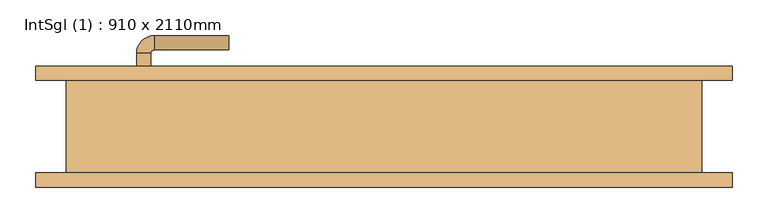
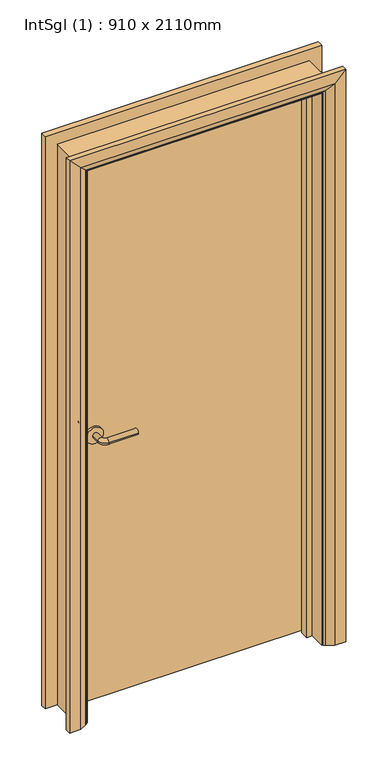
"""IFC4 building model written with IfcOpenShell, lengths in millimetres: door geometry, IntSgl (1) : 910 x 2110mm."""

from ifc_helpers import new_model, si_unit, point, frame, frame_2d, origin, place, context, project, spatial, polyline, circle_curve, ellipse_curve, trimmed, segment, composite_curve, outline, extrude, faceted_brep, source, transform, mapped, element, save
from ifc_brep_helpers import plane_surface, cylinder_surface, revolved_surface, advanced_brep


def intsgl_1_910_x_2110mm_3ac1de32(model_context):
    return source(origin(), model_context, "Body", "SolidModel", [
        advanced_brep(
        [(-348.0, 19.0, 1000.0), (-328.0, 19.0, 1000.0), (-328.0, -11.0, 1000.0), (-348.0, -11.0, 1000.0), (-323.0, -16.0, 1000.0), (-323.0, -36.0, 1000.0), (-218.0, -36.0, 1000.0), (-218.0, -16.0, 1000.0)],
        [
            (0, 1, circle_curve(frame((-338.0, 19.0, 1000.0), z_axis=(0.0, 1.0, 0.0), x_axis=(1.0, 0.0, 0.0)), 10.0)),
            (1, 0, circle_curve(frame((-338.0, 19.0, 1000.0), z_axis=(0.0, 1.0, 0.0), x_axis=(1.0, 0.0, 0.0)), 10.0)),
            (1, 2),
            (2, 3, circle_curve(frame((-338.0, -11.0, 1000.0), z_axis=(0.0, 1.0, 0.0), x_axis=(1.0, 0.0, 0.0)), 10.0)),
            (3, 0),
            (3, 2, circle_curve(frame((-338.0, -11.0, 1000.0), z_axis=(0.0, 1.0, 0.0), x_axis=(1.0, 0.0, 0.0)), 10.0)),
            (4, 5, circle_curve(frame((-323.0, -26.0, 1000.0), z_axis=(-1.0, 0.0, 0.0), x_axis=(0.0, 1.0, 0.0)), 10.0)),
            (5, 3, circle_curve(frame((-323.0, -11.0, 1000.0), z_axis=(0.0, 0.0, -1.0), x_axis=(-1.0, 0.0, 0.0)), 25.0)),
            (2, 4, circle_curve(frame((-323.0, -11.0, 1000.0), z_axis=(0.0, 0.0, 1.0), x_axis=(-1.0, 0.0, 0.0)), 5.0)),
            (5, 4, circle_curve(frame((-323.0, -26.0, 1000.0), z_axis=(-1.0, 0.0, 0.0), x_axis=(0.0, 1.0, 0.0)), 10.0)),
            (6, 7, circle_curve(frame((-218.0, -26.0, 1000.0), z_axis=(1.0, 0.0, 0.0), x_axis=(0.0, 1.0, 0.0)), 10.0)),
            (7, 6, circle_curve(frame((-218.0, -26.0, 1000.0), z_axis=(1.0, 0.0, 0.0), x_axis=(0.0, 1.0, 0.0)), 10.0)),
            (4, 7),
            (6, 5),
        ],
        [
            plane_surface(frame((-338.0, 19.0, 1000.0), z_axis=(0.0, 1.0, 0.0), x_axis=(0.0, 0.0, 1.0))),
            cylinder_surface(frame((-338.0, 19.0, 1000.0), z_axis=(0.0, 1.0, 0.0), x_axis=(1.0, 0.0, 0.0)), 10.0),
            revolved_surface(trimmed(ellipse_curve(frame((-338.0, -11.0, 1000.0), z_axis=(0.0, -1.0, 0.0), x_axis=(1.0, 0.0, 0.0)), 10.0, 10.0), [point((-348.0, -11.0, 1000.0))], [point((-328.0, -11.0, 1000.0))], True, "CARTESIAN"), (-323.0, -11.0, 1000.0), (0.0, 0.0, -1.0)),
            revolved_surface(trimmed(ellipse_curve(frame((-338.0, -11.0, 1000.0), z_axis=(0.0, -1.0, 0.0), x_axis=(1.0, 0.0, 0.0)), 10.0, 10.0), [point((-328.0, -11.0, 1000.0))], [point((-348.0, -11.0, 1000.0))], True, "CARTESIAN"), (-323.0, -11.0, 1000.0), (0.0, 0.0, -1.0)),
            plane_surface(frame((-218.0, -26.0, 1000.0), z_axis=(1.0, 0.0, 0.0), x_axis=(0.0, 0.0, 1.0))),
            cylinder_surface(frame((-323.0, -26.0, 1000.0), z_axis=(-1.0, 0.0, 0.0), x_axis=(0.0, 1.0, 0.0)), 10.0),
        ],
        [
            (0, [[1, 2]]),
            (1, [[3, 4, 5, -2]]),
            (1, [[-5, 6, -3, -1]]),
            (2, [[7, 8, -4, 9]]),
            (3, [[10, -9, -6, -8]]),
            (4, [[11, 12]]),
            (5, [[13, -11, 14, -7]]),
            (5, [[-14, -12, -13, -10]]),
        ],
    ),
        extrude(outline(composite_curve([segment(trimmed(circle_curve(frame_2d((1000.0, -340.5)), 30.0), [point((1000.0, -370.5))], [point((1000.0, -310.5))], False, "CARTESIAN"), True, "CONTINUOUS"), segment(trimmed(circle_curve(frame_2d((1000.0, -340.5)), 30.0), [point((1000.0, -310.5))], [point((1000.0, -370.5))], False, "CARTESIAN"), True, "CONTINUOUS")], self_intersect=False)), frame((0.0, 19.0, 0.0), z_axis=(0.0, 1.0, 0.0), x_axis=(0.0, 0.0, 1.0)), (0.0, 0.0, 1.0), 8.0),
        advanced_brep(
        [(-348.0, 73.0, 1000.0), (-328.0, 73.0, 1000.0), (-348.0, 103.0, 1000.0), (-328.0, 103.0, 1000.0), (-323.0, 108.0, 1000.0), (-323.0, 128.0, 1000.0), (-218.0, 128.0, 1000.0), (-218.0, 108.0, 1000.0)],
        [
            (0, 1, circle_curve(frame((-338.0, 73.0, 1000.0), z_axis=(0.0, -1.0, 0.0), x_axis=(1.0, 0.0, 0.0)), 10.0)),
            (1, 0, circle_curve(frame((-338.0, 73.0, 1000.0), z_axis=(0.0, -1.0, 0.0), x_axis=(1.0, 0.0, 0.0)), 10.0)),
            (0, 2),
            (2, 3, circle_curve(frame((-338.0, 103.0, 1000.0), z_axis=(0.0, -1.0, 0.0), x_axis=(1.0, 0.0, 0.0)), 10.0)),
            (3, 1),
            (3, 2, circle_curve(frame((-338.0, 103.0, 1000.0), z_axis=(0.0, -1.0, 0.0), x_axis=(1.0, 0.0, 0.0)), 10.0)),
            (4, 3, circle_curve(frame((-323.0, 103.0, 1000.0), z_axis=(0.0, 0.0, 1.0), x_axis=(-1.0, 0.0, 0.0)), 5.0)),
            (2, 5, circle_curve(frame((-323.0, 103.0, 1000.0), z_axis=(0.0, 0.0, -1.0), x_axis=(-1.0, 0.0, 0.0)), 25.0)),
            (5, 4, circle_curve(frame((-323.0, 118.0, 1000.0), z_axis=(-1.0, 0.0, 0.0), x_axis=(0.0, -1.0, 0.0)), 10.0)),
            (4, 5, circle_curve(frame((-323.0, 118.0, 1000.0), z_axis=(-1.0, 0.0, 0.0), x_axis=(0.0, -1.0, 0.0)), 10.0)),
            (6, 7, circle_curve(frame((-218.0, 118.0, 1000.0), z_axis=(1.0, 0.0, 0.0), x_axis=(0.0, -1.0, 0.0)), 10.0)),
            (7, 6, circle_curve(frame((-218.0, 118.0, 1000.0), z_axis=(1.0, 0.0, 0.0), x_axis=(0.0, -1.0, 0.0)), 10.0)),
            (5, 6),
            (7, 4),
        ],
        [
            plane_surface(frame((-338.0, 73.0, 1000.0), z_axis=(0.0, -1.0, 0.0), x_axis=(0.0, 0.0, 1.0))),
            cylinder_surface(frame((-338.0, 73.0, 1000.0), z_axis=(0.0, -1.0, 0.0), x_axis=(1.0, 0.0, 0.0)), 10.0),
            revolved_surface(trimmed(ellipse_curve(frame((-338.0, 103.0, 1000.0), z_axis=(0.0, -1.0, 0.0), x_axis=(1.0, 0.0, 0.0)), 10.0, 10.0), [point((-348.0, 103.0, 1000.0))], [point((-328.0, 103.0, 1000.0))], True, "CARTESIAN"), (-323.0, 103.0, 1000.0), (0.0, 0.0, -1.0)),
            revolved_surface(trimmed(ellipse_curve(frame((-338.0, 103.0, 1000.0), z_axis=(0.0, -1.0, 0.0), x_axis=(1.0, 0.0, 0.0)), 10.0, 10.0), [point((-328.0, 103.0, 1000.0))], [point((-348.0, 103.0, 1000.0))], True, "CARTESIAN"), (-323.0, 103.0, 1000.0), (0.0, 0.0, -1.0)),
            plane_surface(frame((-218.0, 118.0, 1000.0), z_axis=(1.0, 0.0, 0.0), x_axis=(0.0, 0.0, 1.0))),
            cylinder_surface(frame((-323.0, 118.0, 1000.0), z_axis=(-1.0, 0.0, 0.0), x_axis=(0.0, -1.0, 0.0)), 10.0),
        ],
        [
            (0, [[1, 2]]),
            (1, [[-1, 3, 4, 5]]),
            (1, [[-2, -5, 6, -3]]),
            (2, [[7, -4, 8, 9]]),
            (3, [[-8, -6, -7, 10]]),
            (4, [[11, 12]]),
            (5, [[-9, 13, -12, 14]]),
            (5, [[-10, -14, -11, -13]]),
        ],
    ),
        extrude(outline(composite_curve([segment(trimmed(circle_curve(frame_2d((1000.0, -340.5)), 30.0), [point((1000.0, -370.5))], [point((1000.0, -310.5))], False, "CARTESIAN"), True, "CONTINUOUS"), segment(trimmed(circle_curve(frame_2d((1000.0, -340.5)), 30.0), [point((1000.0, -310.5))], [point((1000.0, -370.5))], False, "CARTESIAN"), True, "CONTINUOUS")], self_intersect=False)), frame((0.0, 65.0, 0.0), z_axis=(0.0, 1.0, 0.0), x_axis=(0.0, 0.0, 1.0)), (0.0, 0.0, 1.0), 8.0),
        extrude(outline(polyline([(413.0, 27.0), (-413.0, 27.0), (-413.0, 65.0), (413.0, 65.0), (413.0, 27.0)])), frame((0.0, 0.0, 8.0), z_axis=(0.0, 0.0, 1.0), x_axis=(1.0, 0.0, 0.0)), (0.0, 0.0, 1.0), 2060.0),
        advanced_brep(
        [(490.0, 85.0, 0.0), (490.0, 65.0, 0.0), (420.0, 65.0, 0.0), (424.0, 71.0, 0.0), (450.0, 85.0, 0.0), (490.0, 85.0, 2145.0), (490.0, 65.0, 2145.0), (-490.0, 65.0, 2145.0), (-490.0, 65.0, 0.0), (-420.0, 65.0, 0.0), (-420.0, 65.0, 2075.0), (420.0, 65.0, 2075.0), (424.0, 71.0, 2079.0), (450.0, 85.0, 2105.0), (-450.0, 85.0, 2105.0), (-450.0, 85.0, 0.0), (-490.0, 85.0, 0.0), (-490.0, 85.0, 2145.0), (-424.0, 71.0, 2079.0), (-424.0, 71.0, 0.0)],
        [
            (0, 1),
            (1, 2),
            (2, 3, circle_curve(frame((428.0, 64.0, 0.0), z_axis=(0.0, 0.0, -1.0), x_axis=(1.0, 0.0, 0.0)), 8.0622577)),
            (3, 4),
            (4, 0),
            (0, 5),
            (5, 6),
            (6, 1),
            (6, 7),
            (7, 8),
            (8, 9),
            (9, 10),
            (10, 11),
            (11, 2),
            (11, 12, ellipse_curve(frame((428.0, 64.0, 2083.0), z_axis=(0.7071067811865475, 0.0, -0.7071067811865475), x_axis=(-0.7071067811865474, 0.0, -0.7071067811865476)), 11.4017543, 8.0622577)),
            (12, 3),
            (12, 13),
            (13, 4),
            (13, 14),
            (14, 15),
            (15, 16),
            (16, 17),
            (17, 5),
            (17, 7),
            (10, 18, ellipse_curve(frame((-428.0, 64.0, 2083.0), z_axis=(0.7071067811865475, 0.0, 0.7071067811865475), x_axis=(0.7071067811865476, 0.0, -0.7071067811865474)), 11.4017543, 8.0622577)),
            (18, 12),
            (18, 14),
            (15, 19),
            (19, 9, circle_curve(frame((-428.0, 64.0, 0.0), z_axis=(0.0, 0.0, -1.0), x_axis=(-1.0, 0.0, 0.0)), 8.0622577)),
            (8, 16),
            (19, 18),
        ],
        [
            plane_surface(frame((420.0, 65.0, 0.0), z_axis=(0.0, 0.0, -1.0), x_axis=(0.0, -1.0, 0.0))),
            plane_surface(frame((490.0, 85.0, 0.0), z_axis=(1.0, 0.0, 0.0), x_axis=(0.0, 0.0, 1.0))),
            plane_surface(frame((490.0, 65.0, 0.0), z_axis=(0.0, -1.0, 0.0), x_axis=(0.0, 0.0, 1.0))),
            cylinder_surface(frame((428.0, 64.0, 0.0), z_axis=(0.0, 0.0, -1.0), x_axis=(1.0, 0.0, 0.0)), 8.0622577),
            plane_surface(frame((424.0, 71.0, 0.0), z_axis=(-0.4740998230350126, 0.880471099922178, 0.0), x_axis=(0.0, 0.0, 1.0))),
            plane_surface(frame((450.0, 85.0, 0.0), z_axis=(0.0, 1.0, 0.0), x_axis=(0.0, 0.0, 1.0))),
            plane_surface(frame((490.0, 85.0, 2145.0), z_axis=(0.0, 0.0, 1.0), x_axis=(-1.0, 0.0, 0.0))),
            cylinder_surface(frame((420.0, 64.0, 2083.0), z_axis=(1.0, 0.0, 0.0), x_axis=(0.0, 0.0, 1.0)), 8.0622577),
            plane_surface(frame((424.0, 71.0, 2079.0), z_axis=(0.0, 0.8804710999221764, -0.4740998230350154), x_axis=(-1.0, 0.0, 0.0))),
            plane_surface(frame((-420.0, 65.0, 0.0), z_axis=(0.0, 0.0, -1.0), x_axis=(0.0, -1.0, 0.0))),
            plane_surface(frame((-490.0, 85.0, 2145.0), z_axis=(-1.0, 0.0, 0.0), x_axis=(0.0, 0.0, -1.0))),
            cylinder_surface(frame((-428.0, 64.0, 2075.0), z_axis=(0.0, 0.0, 1.0), x_axis=(-1.0, 0.0, 0.0)), 8.0622577),
            plane_surface(frame((-424.0, 71.0, 2079.0), z_axis=(0.47409982303501824, 0.8804710999221749, 0.0), x_axis=(0.0, 0.0, -1.0))),
        ],
        [
            (0, [[1, 2, 3, 4, 5]]),
            (1, [[-1, 6, 7, 8]]),
            (2, [[-2, -8, 9, 10, 11, 12, 13, 14]]),
            (3, [[-3, -14, 15, 16]]),
            (4, [[-4, -16, 17, 18]]),
            (5, [[-5, -18, 19, 20, 21, 22, 23, -6]]),
            (6, [[-7, -23, 24, -9]]),
            (7, [[-15, -13, 25, 26]]),
            (8, [[-17, -26, 27, -19]]),
            (9, [[-21, 28, 29, -11, 30]]),
            (10, [[-24, -22, -30, -10]]),
            (11, [[-25, -12, -29, 31]]),
            (12, [[-27, -31, -28, -20]]),
        ],
    ),
        extrude(outline(polyline([(0.0, -415.0), (0.0, -396.0), (2051.0, -396.0), (2051.0, 396.0), (0.0, 396.0), (0.0, 415.0), (2070.0, 415.0), (2070.0, -415.0), (0.0, -415.0)])), frame((0.0, -7.0, 0.0), z_axis=(0.0, 1.0, 0.0), x_axis=(0.0, 0.0, 1.0)), (0.0, 0.0, 1.0), 32.0),
        advanced_brep(
        [(-490.0, -85.0, 0.0), (-490.0, -65.0, 0.0), (-420.0, -65.0, 0.0), (-424.0, -71.0, 0.0), (-450.0, -85.0, 0.0), (-490.0, -85.0, 2145.0), (-490.0, -65.0, 2145.0), (-420.0, -65.0, 2075.0), (-424.0, -71.0, 2079.0), (-450.0, -85.0, 2105.0), (490.0, -85.0, 2145.0), (490.0, -65.0, 2145.0), (420.0, -65.0, 2075.0), (424.0, -71.0, 2079.0), (450.0, -85.0, 2105.0), (490.0, -85.0, 0.0), (450.0, -85.0, 0.0), (424.0, -71.0, 0.0), (420.0, -65.0, 0.0), (490.0, -65.0, 0.0)],
        [
            (0, 1),
            (1, 2),
            (2, 3, circle_curve(frame((-428.0, -64.0, 0.0), z_axis=(0.0, 0.0, -1.0), x_axis=(-1.0, 0.0, 0.0)), 8.0622577)),
            (3, 4),
            (4, 0),
            (0, 5),
            (5, 6),
            (6, 1),
            (6, 7),
            (7, 2),
            (7, 8, ellipse_curve(frame((-428.0, -64.0, 2083.0), z_axis=(-0.7071067811865475, 0.0, -0.7071067811865475), x_axis=(0.7071067811865474, 0.0, -0.7071067811865476)), 11.4017543, 8.0622577)),
            (8, 3),
            (8, 9),
            (9, 4),
            (9, 5),
            (5, 10),
            (10, 11),
            (11, 6),
            (11, 12),
            (12, 7),
            (12, 13, ellipse_curve(frame((428.0, -64.0, 2083.0), z_axis=(-0.7071067811865475, 0.0, 0.7071067811865475), x_axis=(-0.7071067811865476, 0.0, -0.7071067811865474)), 11.4017543, 8.0622577)),
            (13, 8),
            (13, 14),
            (14, 9),
            (14, 10),
            (15, 16),
            (16, 17),
            (17, 18, circle_curve(frame((428.0, -64.0, 0.0), z_axis=(0.0, 0.0, -1.0), x_axis=(1.0, 0.0, 0.0)), 8.0622577)),
            (18, 19),
            (19, 15),
            (10, 15),
            (19, 11),
            (18, 12),
            (17, 13),
            (16, 14),
        ],
        [
            plane_surface(frame((-420.0, -137.8010989, 0.0), z_axis=(0.0, 0.0, -1.0), x_axis=(1.0, 0.0, 0.0))),
            plane_surface(frame((-490.0, -85.0, 0.0), z_axis=(-1.0, 0.0, 0.0), x_axis=(0.0, 0.0, 1.0))),
            plane_surface(frame((-490.0, -65.0, 0.0), z_axis=(0.0, 1.0, 0.0), x_axis=(0.0, 0.0, 1.0))),
            cylinder_surface(frame((-428.0, -64.0, 0.0), z_axis=(0.0, 0.0, -1.0), x_axis=(-1.0, 0.0, 0.0)), 8.0622577),
            plane_surface(frame((-424.0, -71.0, 0.0), z_axis=(0.4740998230350183, -0.8804710999221749, 0.0), x_axis=(0.0, 0.0, 1.0))),
            plane_surface(frame((-450.0, -85.0, 0.0), z_axis=(0.0, -1.0, 0.0), x_axis=(0.0, 0.0, 1.0))),
            plane_surface(frame((-490.0, -85.0, 2145.0), z_axis=(0.0, 0.0, 1.0), x_axis=(1.0, 0.0, 0.0))),
            plane_surface(frame((-490.0, -65.0, 2145.0), z_axis=(0.0, 1.0, 0.0), x_axis=(1.0, 0.0, 0.0))),
            cylinder_surface(frame((-420.0, -64.0, 2083.0), z_axis=(-1.0, 0.0, 0.0), x_axis=(0.0, 0.0, 1.0)), 8.0622577),
            plane_surface(frame((-424.0, -71.0, 2079.0), z_axis=(0.0, -0.8804710999221749, -0.4740998230350183), x_axis=(1.0, 0.0, 0.0))),
            plane_surface(frame((-450.0, -85.0, 2105.0), z_axis=(0.0, -1.0, 0.0), x_axis=(1.0, 0.0, 0.0))),
            plane_surface(frame((420.0, -137.8010989, 0.0), z_axis=(0.0, 0.0, -1.0), x_axis=(-1.0, 0.0, 0.0))),
            plane_surface(frame((490.0, -85.0, 2145.0), z_axis=(1.0, 0.0, 0.0), x_axis=(0.0, 0.0, -1.0))),
            plane_surface(frame((490.0, -65.0, 2145.0), z_axis=(0.0, 1.0, 0.0), x_axis=(0.0, 0.0, -1.0))),
            cylinder_surface(frame((428.0, -64.0, 2075.0), z_axis=(0.0, 0.0, 1.0), x_axis=(1.0, 0.0, 0.0)), 8.0622577),
            plane_surface(frame((424.0, -71.0, 2079.0), z_axis=(-0.4740998230350183, -0.8804710999221749, 0.0), x_axis=(0.0, 0.0, -1.0))),
            plane_surface(frame((450.0, -85.0, 2105.0), z_axis=(0.0, -1.0, 0.0), x_axis=(0.0, 0.0, -1.0))),
        ],
        [
            (0, [[1, 2, 3, 4, 5]]),
            (1, [[-1, 6, 7, 8]]),
            (2, [[-2, -8, 9, 10]]),
            (3, [[-3, -10, 11, 12]]),
            (4, [[-4, -12, 13, 14]]),
            (5, [[-5, -14, 15, -6]]),
            (6, [[-7, 16, 17, 18]]),
            (7, [[-9, -18, 19, 20]]),
            (8, [[-11, -20, 21, 22]]),
            (9, [[-13, -22, 23, 24]]),
            (10, [[-15, -24, 25, -16]]),
            (11, [[26, 27, 28, 29, 30]]),
            (12, [[-17, 31, -30, 32]]),
            (13, [[-19, -32, -29, 33]]),
            (14, [[-21, -33, -28, 34]]),
            (15, [[-23, -34, -27, 35]]),
            (16, [[-25, -35, -26, -31]]),
        ],
    ),
        faceted_brep([(-415.0, 65.0, 0.0), (-415.0, -65.0, 0.0), (-447.0, -65.0, 0.0), (-447.0, 65.0, 0.0), (-415.0, 65.0, 2070.0), (-415.0, -65.0, 2070.0), (-447.0, -65.0, 2102.0), (-447.0, 65.0, 2102.0), (415.0, 65.0, 2070.0), (415.0, -65.0, 2070.0), (447.0, -65.0, 2102.0), (447.0, 65.0, 2102.0), (415.0, 65.0, 0.0), (447.0, 65.0, 0.0), (447.0, -65.0, 0.0), (415.0, -65.0, 0.0)], [[[0, 1, 2, 3]], [[1, 0, 4, 5]], [[2, 1, 5, 6]], [[3, 2, 6, 7]], [[0, 3, 7, 4]], [[5, 4, 8, 9]], [[6, 5, 9, 10]], [[7, 6, 10, 11]], [[4, 7, 11, 8]], [[12, 13, 14, 15]], [[9, 8, 12, 15]], [[10, 9, 15, 14]], [[11, 10, 14, 13]], [[8, 11, 13, 12]]]),
    ])


if __name__ == "__main__":
    model = new_model("IFC4")
    model_context = context("Model", 3, world=origin())
    ifc_project = project(units=[si_unit("LENGTHUNIT", "METRE", prefix="MILLI")], contexts=[model_context])
    site = spatial("IfcSite", under=ifc_project)
    building = spatial("IfcBuilding", under=site)
    placement = place(None, origin())
    intsgl_1_910_x_2110mm_shape = intsgl_1_910_x_2110mm_3ac1de32(model_context)
    element("IfcDoor", 1, ObjectType="IntSgl (1) : 910 x 2110mm", at=placement, inside=building, context=model_context, shape_type="MappedRepresentation", body=[
        mapped(intsgl_1_910_x_2110mm_shape, transform((0.0, 0.0, 0.0), x_axis=(1.0, 0.0, 0.0), y_axis=(0.0, 1.0, 0.0), z_axis=(0.0, 0.0, 1.0))),
    ])
    save(model, "model.ifc")

# Revit data of these elements
# Type "IntSgl (1) : 910 x 2110mm"
#   Construction Type Id = "MDOOR"
#   Analytic Construction = "Metal"
#   Type Mark = "41"
#   Type Comments = "Internal Single"
#   Operation = "SingleSwingRight"
#   Manufacturer = "Revit"
#   Keynote = "L20"
#   Description = "Internal Single Door"
#   Visual Light Transmittance = 0
#   Solar Heat Gain Coefficient = 0
#   Heat Transfer Coefficient (U) = 3.7021 W/(m²·K)
#   UnderCut = 8 mm
#   Tolerance = 2 mm
#   Thickness = 38 mm
#   Structural Tolerance = 8 mm
#   StopDepth = 32 mm
#   Stop Thickness = 19 mm
#   Rough Width = 910 mm
#   Rough Height = 2110 mm
#   Height to Top Lock Rail = 1000 mm
#   Handle Z Distance = 1000 mm
#   Handle X Distance = 75 mm
#   Frame Thickness = 32 mm
#   Door Panel Width = 826 mm
#   Door Panel Thickness = 38 mm
#   Door Panel Offset = 0 mm
#   Height = 2110 mm
#   Width = 910 mm
#   Door Panel Height = 2060 mm
#   Architrave Setback = 5 mm
#   Function = 0
#   Vis - Ironmongery = yes
#   Material Ironmongery = Door - Handle
#   Material Frame = Door - Frame/Mullion (1)
#   Material Door = Door - Panel
#   Material Architrave = Door - Architrave
#   Wall Closure = (empty or 0)
# Element 1 (IfcDoor, "IntSgl (1) : 910 x 2110mm")
#   Materials on its faces: "Door - Architrave", "Door - Handle", "Door - Frame/Mullion (1)", "Door - Panel"
# Materials
#   "Door - Handle": class "Miscellaneous", colour RGB 0 0 0, transparency 0, Keynote = "P21"
#   "Door - Frame/Mullion (1)": class "Wood", colour RGB 212 179 113, transparency 0, Keynote = "L20", Cost = 0
#   "Door - Panel": class "Wood", colour RGB 210 159 95, transparency 0, Keynote = "L20"
#   "Door - Architrave": class "Wood", colour RGB 154 90 5, transparency 0, Keynote = "P20"
